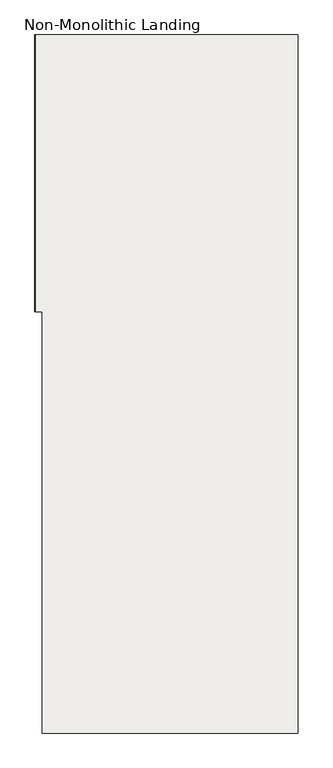
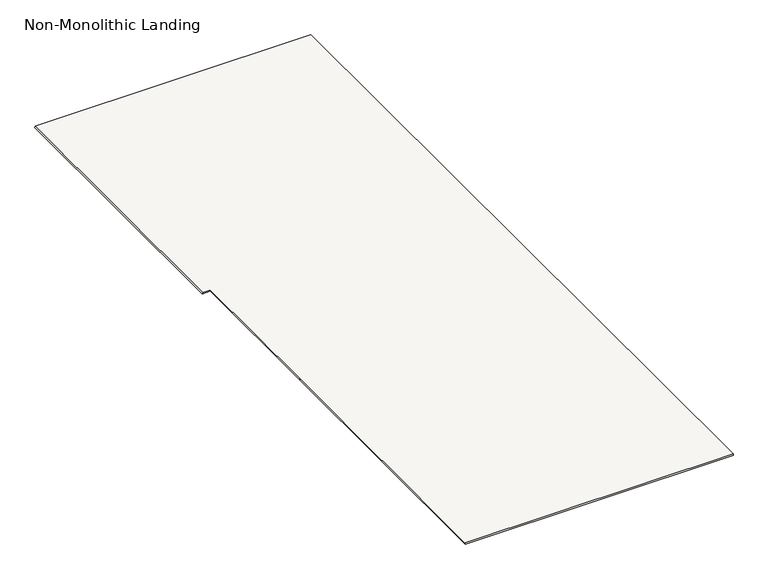
"""IFC4 building model written with IfcOpenShell, lengths in millimetres: slab geometry, Non-Monolithic Landing."""

from ifc_helpers import new_model, si_unit, origin, place, context, project, spatial, faceted_brep, source, transform, mapped, element, save


def non_monolithic_landing_d86126c5(model_context):
    return source(origin(), model_context, "Body", "Brep", [
        faceted_brep([(16318.9400908, 13220.4345331, 30588.2352941), (16318.0900908, 13220.4345331, 30582.2352941), (16318.0900908, 12030.4345331, 30582.2352941), (16318.9400908, 12030.4345331, 30588.2352941), (16350.0, 10220.4345331, 30588.2352941), (17450.0, 10220.4345331, 30588.2352941), (17450.0, 13220.4345331, 30588.2352941), (16350.0, 13220.4345331, 30588.2352941), (16350.0, 12030.4345331, 30588.2352941), (16350.0, 11395.4345331, 30588.2352941), (17450.0, 13220.4345331, 30582.2352941), (17450.0, 10220.4345331, 30582.2352941), (16350.85, 10220.4345331, 30582.2352941), (16350.85, 11395.4345331, 30582.2352941), (16350.0, 11395.4345331, 30582.2352941), (16350.0, 12030.4345331, 30582.2352941), (16350.0, 13220.4345331, 30582.2352941)], [[[0, 1, 2, 3]], [[4, 5, 6, 7, 0, 3, 8, 9]], [[10, 11, 12, 13, 14, 15, 2, 1, 16]], [[9, 8, 15, 14]], [[0, 7, 16, 1]], [[7, 6, 10, 16]], [[6, 5, 11, 10]], [[5, 4, 12, 11]], [[13, 9, 14]], [[9, 13, 12, 4]], [[8, 3, 2, 15]]]),
    ])


if __name__ == "__main__":
    model = new_model("IFC4")
    model_context = context("Model", 3, world=origin())
    ifc_project = project(units=[si_unit("LENGTHUNIT", "METRE", prefix="MILLI")], contexts=[model_context])
    site = spatial("IfcSite", under=ifc_project)
    building = spatial("IfcBuilding", under=site)
    placement = place(None, origin())
    non_monolithic_landing_shape = non_monolithic_landing_d86126c5(model_context)
    element("IfcSlab", 1, ObjectType="Non-Monolithic Landing", at=placement, inside=building, context=model_context, shape_type="MappedRepresentation", body=[
        mapped(non_monolithic_landing_shape, transform((0.0, 0.0, 0.0), x_axis=(1.0, 0.0, 0.0), y_axis=(0.0, 1.0, 0.0), z_axis=(0.0, 0.0, 1.0))),
    ])
    save(model, "model.ifc")

# Revit data of these elements
# Element 1 (IfcSlab, "Non-Monolithic Landing")
#   Materials on its faces: "Steel, Paint Finish, Dark Gray"
# Materials
#   "Steel, Paint Finish, Dark Gray": class "Metal", colour RGB 89 89 89, transparency 0, Description = "Steel, paint finish, dark gray, glossy", Cost = 0
